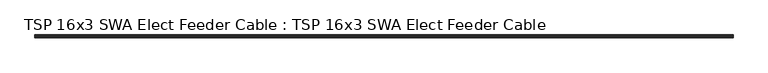
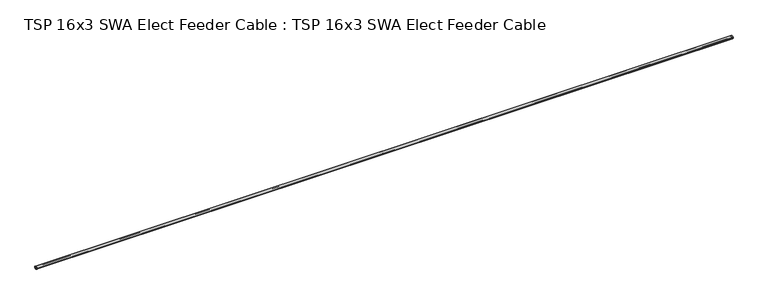
"""IFC4 building model written with IfcOpenShell, lengths in millimetres: proxy geometry, TSP 16x3 SWA Elect Feeder Cable : TSP 16x3 SWA Elect Feeder Cable."""

from ifc_helpers import new_model, si_unit, point, frame, frame_2d, origin, origin_2d, place, context, project, spatial, circle_curve, trimmed, segment, composite_curve, outline, extrude, source, transform, mapped, element, save


def tsp_16x3_swa_elect_feeder_cable_tsp_16x3_swa_elect_feeder_f47cfd59(model_context):
    return source(origin(), model_context, "Body", "SweptSolid", [
        extrude(outline(composite_curve([segment(trimmed(circle_curve(origin_2d(), 30.0), [point((-30.0, 0.0))], [point((30.0, 0.0))], False, "CARTESIAN"), True, "CONTINUOUS"), segment(trimmed(circle_curve(origin_2d(), 30.0), [point((30.0, 0.0))], [point((-30.0, 0.0))], False, "CARTESIAN"), True, "CONTINUOUS")], self_intersect=False), holes=[composite_curve([segment(trimmed(circle_curve(origin_2d(), 27.0), [point((-27.0, 0.0))], [point((27.0, 0.0))], True, "CARTESIAN"), True, "CONTINUOUS"), segment(trimmed(circle_curve(origin_2d(), 27.0), [point((27.0, 0.0))], [point((-27.0, 0.0))], True, "CARTESIAN"), True, "CONTINUOUS")], self_intersect=False)]), frame((0.0, 0.0, 0.0), z_axis=(1.0, 0.0, 0.0), x_axis=(0.0, 1.0, 0.0)), (0.0, 0.0, 1.0), 14700.0),
        extrude(outline(composite_curve([segment(trimmed(circle_curve(frame_2d((11.691343, 6.75)), 8.0), [point((3.691343, 6.75))], [point((19.691343, 6.75))], False, "CARTESIAN"), True, "CONTINUOUS"), segment(trimmed(circle_curve(frame_2d((11.691343, 6.75)), 8.0), [point((19.691343, 6.75))], [point((3.691343, 6.75))], False, "CARTESIAN"), True, "CONTINUOUS")], self_intersect=False)), frame((0.0, 0.0, 0.0), z_axis=(1.0, 0.0, 0.0), x_axis=(0.0, 1.0, 0.0)), (0.0, 0.0, 1.0), 14700.0),
        extrude(outline(composite_curve([segment(trimmed(circle_curve(frame_2d((-11.691343, 6.75)), 8.0), [point((-19.691343, 6.75))], [point((-3.691343, 6.75))], False, "CARTESIAN"), True, "CONTINUOUS"), segment(trimmed(circle_curve(frame_2d((-11.691343, 6.75)), 8.0), [point((-3.691343, 6.75))], [point((-19.691343, 6.75))], False, "CARTESIAN"), True, "CONTINUOUS")], self_intersect=False)), frame((0.0, 0.0, 0.0), z_axis=(1.0, 0.0, 0.0), x_axis=(0.0, 1.0, 0.0)), (0.0, 0.0, 1.0), 14700.0),
        extrude(outline(composite_curve([segment(trimmed(circle_curve(frame_2d((0.0, -13.5)), 8.0), [point((-8.0, -13.5))], [point((8.0, -13.5))], False, "CARTESIAN"), True, "CONTINUOUS"), segment(trimmed(circle_curve(frame_2d((0.0, -13.5)), 8.0), [point((8.0, -13.5))], [point((-8.0, -13.5))], False, "CARTESIAN"), True, "CONTINUOUS")], self_intersect=False)), frame((0.0, 0.0, 0.0), z_axis=(1.0, 0.0, 0.0), x_axis=(0.0, 1.0, 0.0)), (0.0, 0.0, 1.0), 14700.0),
        extrude(outline(composite_curve([segment(trimmed(circle_curve(origin_2d(), 27.0), [point((27.0, 0.0))], [point((-27.0, 0.0))], False, "CARTESIAN"), True, "CONTINUOUS"), segment(trimmed(circle_curve(origin_2d(), 27.0), [point((-27.0, 0.0))], [point((27.0, 0.0))], False, "CARTESIAN"), True, "CONTINUOUS")], self_intersect=False), holes=[composite_curve([segment(trimmed(circle_curve(frame_2d((-11.691343, 6.75)), 8.0), [point((-3.691343, 6.75))], [point((-19.691343, 6.75))], True, "CARTESIAN"), True, "CONTINUOUS"), segment(trimmed(circle_curve(frame_2d((-11.691343, 6.75)), 8.0), [point((-19.691343, 6.75))], [point((-3.691343, 6.75))], True, "CARTESIAN"), True, "CONTINUOUS")], self_intersect=False), composite_curve([segment(trimmed(circle_curve(frame_2d((11.691343, 6.75)), 8.0), [point((3.691343, 6.75))], [point((19.691343, 6.75))], True, "CARTESIAN"), True, "CONTINUOUS"), segment(trimmed(circle_curve(frame_2d((11.691343, 6.75)), 8.0), [point((19.691343, 6.75))], [point((3.691343, 6.75))], True, "CARTESIAN"), True, "CONTINUOUS")], self_intersect=False), composite_curve([segment(trimmed(circle_curve(frame_2d((0.0, -13.5)), 8.0), [point((-8.0, -13.5))], [point((8.0, -13.5))], True, "CARTESIAN"), True, "CONTINUOUS"), segment(trimmed(circle_curve(frame_2d((0.0, -13.5)), 8.0), [point((8.0, -13.5))], [point((-8.0, -13.5))], True, "CARTESIAN"), True, "CONTINUOUS")], self_intersect=False)]), frame((0.0, 0.0, 0.0), z_axis=(1.0, 0.0, 0.0), x_axis=(0.0, 1.0, 0.0)), (0.0, 0.0, 1.0), 14700.0),
    ])


if __name__ == "__main__":
    model = new_model("IFC4")
    model_context = context("Model", 3, world=origin())
    ifc_project = project(units=[si_unit("LENGTHUNIT", "METRE", prefix="MILLI")], contexts=[model_context])
    site = spatial("IfcSite", under=ifc_project)
    building = spatial("IfcBuilding", under=site)
    placement = place(None, origin())
    tsp_16x3_swa_elect_feeder_cable_tsp_16x3_swa_elect_feeder_shape = tsp_16x3_swa_elect_feeder_cable_tsp_16x3_swa_elect_feeder_f47cfd59(model_context)
    element("IfcBuildingElementProxy", 1, Name="TSP 16x3 SWA Elect Feeder Cable : TSP 16x3 SWA Elect Feeder Cable", ObjectType="TSP 16x3 SWA Elect Feeder Cable : TSP 16x3 SWA Elect Feeder Cable", at=placement, inside=building, context=model_context, shape_type="MappedRepresentation", body=[
        mapped(tsp_16x3_swa_elect_feeder_cable_tsp_16x3_swa_elect_feeder_shape, transform((0.0, 0.0, 0.0), x_axis=(1.0, 0.0, 0.0), y_axis=(0.0, 1.0, 0.0), z_axis=(0.0, 0.0, 1.0))),
    ])
    save(model, "model.ifc")

# Revit data of these elements
# Type "TSP 16x3 SWA Elect Feeder Cable : TSP 16x3 SWA Elect Feeder Cable"
#   Model = "TSP_ELECSC163"
#   built-in parameter 1001306 [instance default] = 3.93701 (stored number, unit not read)
#   Cable Length [instance default] = 1200 mm
#   Default Elevation = 0
# Element 1 (IfcBuildingElementProxy, "TSP 16x3 SWA Elect Feeder Cable : TSP 16x3 SWA Elect Feeder Cable")
#   built-in parameter 1001306 = 48.2283 (stored number, unit not read)
#   Cable Length = 14700 mm
#   Materials on its faces: "Cellulose Fill", "Copper", "Laminate, Red, Matte"
# Materials
#   "Cellulose Fill": class "Generic", colour RGB 0 0 0, transparency 0, Description = "Cellulose loose fill", Cost = 0
#   "Copper": class "Metal", colour RGB 0 0 0, transparency 0, Description = "Copper, matte finish", Cost = 0
#   "Laminate, Red, Matte": class "Plastic", colour RGB 255 0 0, transparency 0, Description = "Plastic Laminate - Red, Matte", Cost = 0
